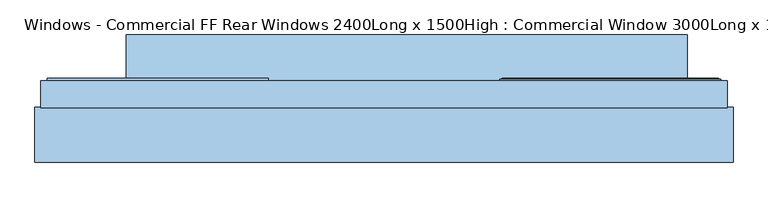
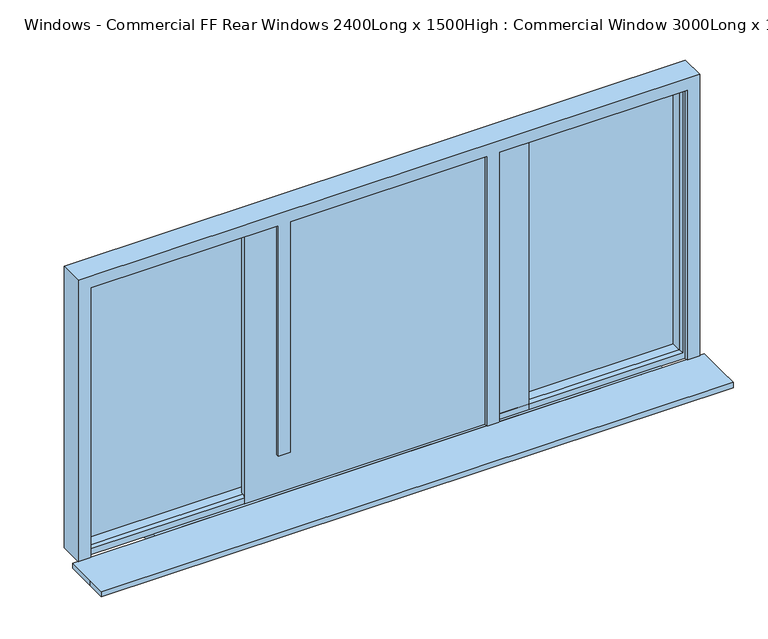
"""IFC4 building model written with IfcOpenShell, lengths in millimetres: window geometry, Windows - Commercial FF Rear Windows 2400Long x 1500High : Commercial Window 3000Long x 1500High 2."""

from ifc_helpers import new_model, si_unit, frame, origin, place, context, project, spatial, polyline, outline, extrude, faceted_brep, source, transform, mapped, element, save


def windows_commercial_ff_rear_windows_2400long_x_1500high_ec56d910(model_context):
    return source(origin(), model_context, "Body", "SolidModel", [
        extrude(outline(polyline([(-2260.0, -231.5434322), (-2260.0, -138.5434322), (-2260.0, 8.4565678), (790.0, 8.4565678), (790.0, -138.5434322), (790.0, -231.5434322), (-2260.0, -231.5434322)])), frame((0.0, 0.0, 636.5715519), z_axis=(0.0, 0.0, 1.0), x_axis=(1.0, 0.0, 0.0)), (0.0, 0.0, 1.0), 26.4284481),
        extrude(outline(polyline([(695.0, 87.4565678), (-190.0, 87.4565678), (-190.0, 111.4565678), (695.0, 111.4565678), (695.0, 87.4565678)])), frame((0.0, 0.0, 693.0), z_axis=(0.0, 0.0, 1.0), x_axis=(1.0, 0.0, 0.0)), (0.0, 0.0, 1.0), 1337.0),
        extrude(outline(polyline([(-1420.0, 47.4565678), (-50.0, 47.4565678), (-50.0, 23.4565678), (-1420.0, 23.4565678), (-1420.0, 47.4565678)])), frame((0.0, 0.0, 663.0), z_axis=(0.0, 0.0, 1.0), x_axis=(1.0, 0.0, 0.0)), (0.0, 0.0, 1.0), 1397.0),
        extrude(outline(polyline([(-1280.0, 87.4565678), (-2165.0, 87.4565678), (-2165.0, 111.4565678), (-1280.0, 111.4565678), (-1280.0, 87.4565678)])), frame((0.0, 0.0, 693.0), z_axis=(0.0, 0.0, 1.0), x_axis=(1.0, 0.0, 0.0)), (0.0, 0.0, 1.0), 1337.0),
        faceted_brep([(-2235.0, 5.4565678, 663.0), (-2175.0, 5.4565678, 663.0), (-2175.0, 5.4565678, 2040.0), (-1268.0, 5.4565678, 2040.0), (-1268.0, 5.4565678, 863.0), (-1210.0, 5.4565678, 863.0), (-1210.0, 5.4565678, 2040.0), (-260.0, 5.4565678, 2040.0), (-260.0, 5.4565678, 663.0), (-202.0, 5.4565678, 663.0), (-202.0, 5.4565678, 2040.0), (705.0, 5.4565678, 2040.0), (705.0, 5.4565678, 663.0), (765.0, 5.4565678, 663.0), (765.0, 5.4565678, 2100.0), (-2235.0, 5.4565678, 2100.0), (-2235.0, 123.4565678, 663.0), (-2235.0, 123.4565678, 2100.0), (-2195.0, 123.4565678, 663.0), (765.0, 123.4565678, 2100.0), (765.0, 123.4565678, 663.0), (725.0, 123.4565678, 663.0), (725.0, 123.4565678, 2060.0), (-220.0, 123.4565678, 2060.0), (-220.0, 123.4565678, 663.0), (-260.0, 123.4565678, 663.0), (-260.0, 123.4565678, 2060.0), (-1210.0, 123.4565678, 2060.0), (-1210.0, 123.4565678, 863.0), (-1250.0, 123.4565678, 863.0), (-1250.0, 123.4565678, 2060.0), (-2195.0, 123.4565678, 2060.0), (-2195.0, 23.4565678, 663.0), (-2195.0, 23.4565678, 2060.0), (-2175.0, 23.4565678, 663.0), (-1250.0, 23.4565678, 2060.0), (-1250.0, 23.4565678, 863.0), (-1268.0, 23.4565678, 863.0), (-1268.0, 23.4565678, 2040.0), (-2175.0, 23.4565678, 2040.0), (725.0, 23.4565678, 2060.0), (725.0, 23.4565678, 663.0), (705.0, 23.4565678, 663.0), (705.0, 23.4565678, 2040.0), (-202.0, 23.4565678, 2040.0), (-202.0, 23.4565678, 663.0), (-220.0, 23.4565678, 663.0), (-220.0, 23.4565678, 2060.0), (-1210.0, 23.4565678, 863.0), (-1220.0, 23.4565678, 863.0), (-1220.0, 23.4565678, 2060.0), (-250.0, 23.4565678, 2060.0), (-250.0, 23.4565678, 663.0), (-260.0, 23.4565678, 663.0), (-260.0, 23.4565678, 2040.0), (-1210.0, 23.4565678, 2040.0), (-1210.0, 47.4565678, 2060.0), (-260.0, 47.4565678, 2060.0), (-250.0, 47.4565678, 2060.0), (-1220.0, 47.4565678, 2060.0), (-1210.0, 47.4565678, 863.0), (-1220.0, 47.4565678, 863.0), (-250.0, 47.4565678, 663.0), (-260.0, 47.4565678, 663.0), (-260.0, 73.4565678, 663.0), (-220.0, 73.4565678, 663.0), (-202.0, 8.4565678, 663.0), (-260.0, 8.4565678, 663.0), (590.0, 323.4565678, 600.0), (590.0, 8.4565678, 600.0), (-1860.0, 8.4565678, 600.0), (-1860.0, 323.4565678, 600.0), (590.0, 323.4565678, 637.0666405), (-1860.0, 323.4565678, 637.0666405), (590.0, 73.4565678, 649.0962075), (-1860.0, 73.4565678, 649.0962075), (590.0, 8.4565678, 663.0), (590.0, 73.4565678, 663.0), (-1860.0, 73.4565678, 663.0), (-1860.0, 8.4565678, 663.0)], [[[0, 1, 2, 3, 4, 5, 6, 7, 8, 9, 10, 11, 12, 13, 14, 15]], [[16, 0, 15, 17]], [[18, 16, 17, 19, 20, 21, 22, 23, 24, 25, 26, 27, 28, 29, 30, 31]], [[32, 18, 31, 33]], [[34, 32, 33, 35, 36, 37, 38, 39]], [[40, 41, 42, 43, 44, 45, 46, 47]], [[48, 49, 50, 51, 52, 53, 54, 55]], [[1, 34, 39, 2]], [[15, 14, 19, 17]], [[33, 31, 30, 35]], [[22, 40, 47, 23]], [[56, 27, 26, 57, 58, 51, 50, 59]], [[2, 39, 38, 3]], [[43, 11, 10, 44]], [[6, 55, 54, 7]], [[14, 13, 20, 19]], [[22, 21, 41, 40]], [[12, 11, 43, 42]], [[5, 48, 55, 6]], [[37, 4, 3, 38]], [[29, 36, 35, 30]], [[60, 28, 27, 56]], [[61, 60, 56, 59]], [[49, 61, 59, 50]], [[58, 62, 52, 51]], [[62, 58, 57, 63]], [[63, 57, 26, 25, 64]], [[24, 23, 47, 46, 65]], [[10, 9, 66, 45, 44]], [[8, 7, 54, 53, 67]], [[68, 69, 70, 71]], [[72, 68, 71, 73]], [[74, 72, 73, 75]], [[76, 77, 65, 46, 45, 66]], [[78, 79, 67, 53, 52, 62, 63, 64]], [[1, 0, 16, 18, 32, 34]], [[13, 12, 42, 41, 21, 20]], [[48, 5, 4, 37, 36, 29, 28, 60, 61, 49]], [[25, 24, 65, 64]], [[9, 8, 67, 66]], [[76, 69, 68, 72, 74, 77]], [[79, 78, 75, 73, 71, 70]], [[77, 74, 75, 78, 64, 65]], [[69, 76, 66, 67, 79, 70]]]),
        faceted_brep([(-1250.0, 23.4565678, 2060.0), (-1250.0, 93.4565678, 2060.0), (-2195.0, 93.4565678, 2060.0), (-2195.0, 23.4565678, 2060.0), (-1290.0, 37.9494677, 2020.0), (-1279.8519623, 23.4565678, 2030.1480377), (-2165.1480377, 23.4565678, 2030.1480377), (-2155.0, 37.9494677, 2020.0), (-1290.0, 87.4565678, 2020.0), (-2155.0, 87.4565678, 2020.0), (-1280.0, 111.4565678, 2030.0), (-1280.0, 87.4565678, 2030.0), (-2165.0, 87.4565678, 2030.0), (-2165.0, 111.4565678, 2030.0), (-1290.0, 129.2300705, 2020.0), (-1290.0, 111.4565678, 2020.0), (-2155.0, 111.4565678, 2020.0), (-2155.0, 129.2300705, 2020.0), (-1271.1854344, 135.0035732, 2038.8145656), (-2173.8145656, 135.0035732, 2038.8145656), (-2195.0, 93.4565678, 663.0), (-2195.0, 23.4565678, 663.0), (-2165.1480377, 23.4565678, 692.8519623), (-2155.0, 37.9494677, 703.0), (-2155.0, 87.4565678, 703.0), (-2165.0, 87.4565678, 693.0), (-2165.0, 111.4565678, 693.0), (-2155.0, 111.4565678, 703.0), (-2155.0, 129.2300705, 703.0), (-2173.8145656, 135.0035732, 684.1854344), (-1250.0, 93.4565678, 663.0), (-1250.0, 23.4565678, 663.0), (-1279.8519623, 23.4565678, 692.8519623), (-1290.0, 37.9494677, 703.0), (-1290.0, 87.4565678, 703.0), (-1280.0, 87.4565678, 693.0), (-1280.0, 111.4565678, 693.0), (-1290.0, 111.4565678, 703.0), (-1290.0, 129.2300705, 703.0), (-1271.1854344, 135.0035732, 684.1854344), (-1240.0, 135.0035732, 653.0), (-2205.0, 135.0035732, 653.0), (-2205.0, 135.0035732, 2070.0), (-1240.0, 135.0035732, 2070.0), (-1240.0, 93.4565678, 2070.0), (-2205.0, 93.4565678, 2070.0), (-2205.0, 93.4565678, 653.0), (-1240.0, 93.4565678, 653.0)], [[[0, 1, 2, 3]], [[4, 5, 6, 7]], [[8, 4, 7, 9]], [[10, 11, 12, 13]], [[14, 15, 16, 17]], [[18, 14, 17, 19]], [[3, 2, 20, 21]], [[7, 6, 22, 23]], [[9, 7, 23, 24]], [[13, 12, 25, 26]], [[17, 16, 27, 28]], [[19, 17, 28, 29]], [[21, 20, 30, 31]], [[0, 3, 21, 31], [32, 22, 6, 5]], [[23, 22, 32, 33]], [[24, 23, 33, 34]], [[35, 25, 12, 11], [8, 9, 24, 34]], [[26, 25, 35, 36]], [[10, 13, 26, 36], [37, 27, 16, 15]], [[28, 27, 37, 38]], [[29, 28, 38, 39]], [[40, 41, 42, 43], [18, 19, 29, 39]], [[30, 1, 0, 31]], [[33, 32, 5, 4]], [[34, 33, 4, 8]], [[36, 35, 11, 10]], [[38, 37, 15, 14]], [[39, 38, 14, 18]], [[44, 43, 42, 45]], [[45, 42, 41, 46]], [[46, 41, 40, 47]], [[47, 40, 43, 44]], [[45, 46, 47, 44], [1, 30, 20, 2]]]),
        faceted_brep([(-230.0, 87.4565678, 2070.0), (-230.0, 129.2300705, 2070.0), (-230.0, 129.2300705, 653.0), (-230.0, 87.4565678, 653.0), (-220.0, 23.4565678, 2060.0), (-220.0, 87.4565678, 2060.0), (-220.0, 87.4565678, 663.0), (-220.0, 23.4565678, 663.0), (-180.0, 37.9494677, 2020.0), (-190.1480377, 23.4565678, 2030.1480377), (-190.1480377, 23.4565678, 692.8519623), (-180.0, 37.9494677, 703.0), (-180.0, 87.4565678, 2020.0), (-180.0, 87.4565678, 703.0), (-190.0, 111.4565678, 2030.0), (-190.0, 87.4565678, 2030.0), (-190.0, 87.4565678, 693.0), (-190.0, 111.4565678, 693.0), (-180.0, 129.2300705, 2020.0), (-180.0, 111.4565678, 2020.0), (-180.0, 111.4565678, 703.0), (-180.0, 129.2300705, 703.0), (-197.4457548, 135.0035732, 2037.4457548), (-197.4457548, 135.0035732, 685.5542452), (-219.2153903, 135.0035732, 2059.2153903), (-219.2153903, 135.0035732, 663.7846097), (735.0, 129.2300705, 653.0), (735.0, 87.4565678, 653.0), (725.0, 87.4565678, 663.0), (725.0, 23.4565678, 663.0), (695.1480377, 23.4565678, 692.8519623), (685.0, 37.9494677, 703.0), (685.0, 87.4565678, 703.0), (695.0, 87.4565678, 693.0), (695.0, 111.4565678, 693.0), (685.0, 111.4565678, 703.0), (685.0, 129.2300705, 703.0), (702.4457548, 135.0035732, 685.5542452), (724.2153903, 135.0035732, 663.7846097), (735.0, 129.2300705, 2070.0), (735.0, 87.4565678, 2070.0), (725.0, 87.4565678, 2060.0), (725.0, 23.4565678, 2060.0), (695.1480377, 23.4565678, 2030.1480377), (685.0, 37.9494677, 2020.0), (685.0, 87.4565678, 2020.0), (695.0, 87.4565678, 2030.0), (695.0, 111.4565678, 2030.0), (685.0, 111.4565678, 2020.0), (685.0, 129.2300705, 2020.0), (702.4457548, 135.0035732, 2037.4457548), (724.2153903, 135.0035732, 2059.2153903)], [[[0, 1, 2, 3]], [[4, 5, 6, 7]], [[8, 9, 10, 11]], [[12, 8, 11, 13]], [[14, 15, 16, 17]], [[18, 19, 20, 21]], [[22, 18, 21, 23]], [[1, 24, 25, 2]], [[3, 2, 26, 27]], [[7, 6, 28, 29]], [[11, 10, 30, 31]], [[13, 11, 31, 32]], [[17, 16, 33, 34]], [[21, 20, 35, 36]], [[23, 21, 36, 37]], [[2, 25, 38, 26]], [[27, 26, 39, 40]], [[29, 28, 41, 42]], [[31, 30, 43, 44]], [[32, 31, 44, 45]], [[34, 33, 46, 47]], [[36, 35, 48, 49]], [[37, 36, 49, 50]], [[26, 38, 51, 39]], [[40, 39, 1, 0]], [[42, 41, 5, 4]], [[7, 29, 42, 4], [9, 43, 30, 10]], [[44, 43, 9, 8]], [[45, 44, 8, 12]], [[15, 46, 33, 16], [13, 32, 45, 12]], [[47, 46, 15, 14]], [[17, 34, 47, 14], [19, 48, 35, 20]], [[49, 48, 19, 18]], [[50, 49, 18, 22]], [[24, 51, 38, 25], [23, 37, 50, 22]], [[39, 51, 24, 1]], [[3, 27, 40, 0], [5, 41, 28, 6]]]),
    ])


if __name__ == "__main__":
    model = new_model("IFC4")
    model_context = context("Model", 3, world=origin())
    ifc_project = project(units=[si_unit("LENGTHUNIT", "METRE", prefix="MILLI")], contexts=[model_context])
    site = spatial("IfcSite", under=ifc_project)
    building = spatial("IfcBuilding", under=site)
    placement = place(None, origin())
    windows_commercial_ff_rear_windows_2400long_x_1500high_shape = windows_commercial_ff_rear_windows_2400long_x_1500high_ec56d910(model_context)
    element("IfcWindow", 1, ObjectType="Windows - Commercial FF Rear Windows 2400Long x 1500High : Commercial Window 3000Long x 1500High 2", at=placement, inside=building, context=model_context, shape_type="MappedRepresentation", body=[
        mapped(windows_commercial_ff_rear_windows_2400long_x_1500high_shape, transform((0.0, 0.0, 0.0), x_axis=(1.0, 0.0, 0.0), y_axis=(0.0, 1.0, 0.0), z_axis=(0.0, 0.0, 1.0))),
    ])
    save(model, "model.ifc")

# Revit data of these elements
# Type "Windows - Commercial FF Rear Windows 2400Long x 1500High : Commercial Window 3000Long x 1500High 2"
#   Type Mark = "67"
#   Operation = "Triple Panel Vertical"
#   Description = "Double Glazed First Floor Window"
#   Manufacturer = "aluminium Co"
#   Keynote = "L10"
#   Wrap Layers (Ext) from Ext = 100 mm
#   Wrap Layers (Int) from Ext = 177.5 mm
#   Window Board Projection = 25 mm
#   Window Board Extension = 25 mm
#   Visual Light Transmittance = 0.9
#   Solar Heat Gain Coefficient = 0.78
#   Rough Width = 3000 mm
#   Rough Height = 1500 mm
#   Height = 1500 mm
#   Width = 3000 mm
#   Heat Transfer Coefficient (U) = 3.6886 W/(m²·K)
#   Glazing Thickness = 24 mm
#   FrameOffset - External = 100 mm
#   Frame Depth = 100 mm
#   Default Head Height = 2100 mm
#   Cill Depth = 200 mm
#   Cavity Closer Width = 100 mm
#   Cavity Closer Offset from Ext = 130 mm
#   Cavity Closer Depth = 85 mm
#   Vis - Cavity Closers = yes
#   Define Thermal Properties by = 1
#   Material Trim = Window Frame
#   Material Glass = Glass
#   Material Frame = Window Frame
#   Construction Type Id = ""
#   Wall Closure = (empty or 0)
#   Analytic Construction = (empty or 0)
# Element 1 (IfcWindow, "Windows - Commercial FF Rear Windows 2400Long x 1500High : Commercial Window 3000Long x 1500High 2")
#   Materials on its faces: "Window Frame", "Glass"
# Materials
#   "Window Frame": class "Miscellaneous", colour RGB 249 249 249, transparency 0, Keynote = "L10"
#   "Glass": class "Glass", colour RGB 0 128 192, transparency 0.9, Description = "Soda Lime Glass", Cost = 0
